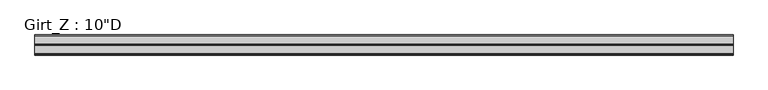
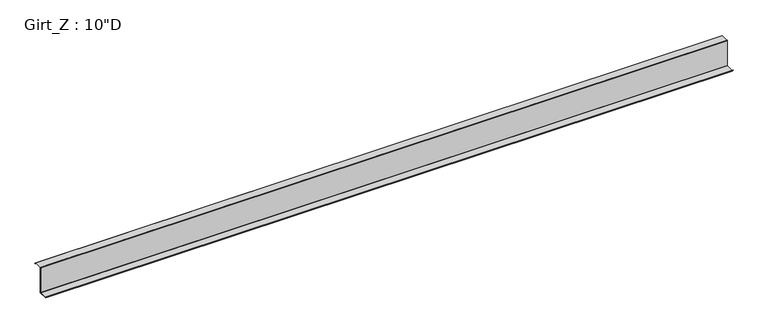
"""IFC4 building model written with IfcOpenShell, lengths in millimetres: beam geometry."""

import ifcopenshell
import ifcopenshell.guid

model = None  # the IFC model being written
_history = None  # IfcOwnerHistory: only IFC2X3 demands one
_inside = {}  # id of a spatial element -> (the spatial element, [elements in it])
_under = {}  # id of a project, library or spatial element -> (it, [spatial elements below it])
_declared = {}  # id of a project -> (the project, [libraries it declares])
_typed = {}  # id of a type object -> (the type object, [elements of that type])
_made_of = {}  # id of a material, layer set ... -> (it, [elements and type objects made of it])


def new_model(schema):
    """Start an empty IFC model of exactly this schema.

    Asked for "IFC4X3", IfcOpenShell would pick the latest addendum, in which some entities
    have other attributes; the version numbers below select the first issue.
    IFC2X3 requires an IfcOwnerHistory on every rooted entity: one is made here for all.
    """
    global model, _history
    if schema == "IFC4X3":
        model = ifcopenshell.file(schema_version=(4, 3, 0, 0))
    else:
        model = ifcopenshell.file(schema=schema)
    _inside.clear()
    _under.clear()
    _declared.clear()
    _typed.clear()
    _made_of.clear()
    _history = None
    if model.schema == "IFC2X3":
        org = make("IfcOrganization", Name="unknown")
        user = make(
            "IfcPersonAndOrganization",
            ThePerson=make("IfcPerson", FamilyName="unknown"),
            TheOrganization=org,
        )
        app = make(
            "IfcApplication",
            ApplicationDeveloper=org,
            Version="unknown",
            ApplicationFullName="unknown",
            ApplicationIdentifier="unknown",
        )
        _history = make(
            "IfcOwnerHistory",
            OwningUser=user,
            OwningApplication=app,
            ChangeAction="ADDED",
            CreationDate=0,
        )
    return model


def make(cls, **values):
    """One entity of the class cls with the attributes given. An attribute that is None is left unset."""
    return model.create_entity(
        cls, **{name: value for name, value in values.items() if value is not None}
    )


def rooted(cls, **values):
    """An entity with a GlobalId (a new one), such as an element, a storey or a relation."""
    return make(cls, GlobalId=ifcopenshell.guid.new(), OwnerHistory=_history, **values)


def si_unit(unit_type, name, prefix=None):
    """IfcSIUnit, for example si_unit("LENGTHUNIT", "METRE", prefix="MILLI")."""
    return make("IfcSIUnit", UnitType=unit_type, Prefix=prefix, Name=name)


def assignment(units):
    """IfcUnitAssignment: the units of a project."""
    return None if units is None else make("IfcUnitAssignment", Units=units)


def point(xyz):
    """IfcCartesianPoint."""
    return None if xyz is None else make("IfcCartesianPoint", Coordinates=xyz)


def direction(xyz):
    """IfcDirection."""
    return None if xyz is None else make("IfcDirection", DirectionRatios=xyz)


def frame(location, z_axis=None, x_axis=None):
    """IfcAxis2Placement3D, a coordinate frame: its origin and axes. An axis left out is left unset."""
    return make(
        "IfcAxis2Placement3D",
        Location=point(location),
        Axis=direction(z_axis),
        RefDirection=direction(x_axis),
    )


def frame_2d(location, x_axis=None):
    """IfcAxis2Placement2D, a coordinate frame in the plane: its origin and x axis."""
    return make(
        "IfcAxis2Placement2D", Location=point(location), RefDirection=direction(x_axis)
    )


def origin():
    """The frame at (0, 0, 0) with its axes left unset."""
    return frame((0.0, 0.0, 0.0))


def place(relative_to, where):
    """IfcLocalPlacement: puts the frame where relative to a parent placement (None: the world)."""
    return make(
        "IfcLocalPlacement", PlacementRelTo=relative_to, RelativePlacement=where
    )


def context(
    kind, dimensions, precision=None, world=None, true_north=None, identifier=None
):
    """IfcGeometricRepresentationContext, for example the 3D "Model" context."""
    return make(
        "IfcGeometricRepresentationContext",
        ContextIdentifier=identifier,
        ContextType=kind,
        CoordinateSpaceDimension=dimensions,
        Precision=precision,
        WorldCoordinateSystem=world,
        TrueNorth=true_north,
    )


def project(units=None, contexts=None):
    """IfcProject with its units and contexts."""
    return rooted(
        "IfcProject",
        Name="project",
        RepresentationContexts=contexts,
        UnitsInContext=assignment(units),
    )


def spatial(cls, under=None, at=None, **own):
    """A site, building, storey or space (cls), placed at a placement, below another one or the project."""
    s = rooted(cls, ObjectPlacement=at, **own)
    if under is not None:
        _under.setdefault(under.id(), (under, []))[1].append(s)
    return s


def polyline(points):
    """IfcPolyline through the points."""
    return make("IfcPolyline", Points=[point(p) for p in points])


def circle_curve(where, radius):
    """IfcCircle in the frame where."""
    return make("IfcCircle", Position=where, Radius=radius)


def trimmed(basis, trim1, trim2, sense, master):
    """IfcTrimmedCurve: the piece of a basis curve between two trims."""
    return make(
        "IfcTrimmedCurve",
        BasisCurve=basis,
        Trim1=trim1,
        Trim2=trim2,
        SenseAgreement=sense,
        MasterRepresentation=master,
    )


def segment(curve, same_sense, transition):
    """IfcCompositeCurveSegment."""
    return make(
        "IfcCompositeCurveSegment",
        Transition=transition,
        SameSense=same_sense,
        ParentCurve=curve,
    )


def composite_curve(segments, self_intersect=None):
    """IfcCompositeCurve: segments joined end to end."""
    return make("IfcCompositeCurve", Segments=segments, SelfIntersect=self_intersect)


def outline(outer, holes=None, kind="AREA"):
    """IfcArbitraryClosedProfileDef: a profile drawn as a closed curve; with holes, ...WithVoids."""
    if holes is None:
        return make("IfcArbitraryClosedProfileDef", ProfileType=kind, OuterCurve=outer)
    return make(
        "IfcArbitraryProfileDefWithVoids",
        ProfileType=kind,
        OuterCurve=outer,
        InnerCurves=holes,
    )


def extrude(swept, where, along, depth):
    """IfcExtrudedAreaSolid: the profile swept, set in the frame where, extruded along a direction by depth."""
    return make(
        "IfcExtrudedAreaSolid",
        SweptArea=swept,
        Position=where,
        ExtrudedDirection=direction(along),
        Depth=depth,
    )


def shape(context_of_items, identifier, shape_type, items):
    """IfcShapeRepresentation: the items that make up one representation, for example the "Body"."""
    return make(
        "IfcShapeRepresentation",
        ContextOfItems=context_of_items,
        RepresentationIdentifier=identifier,
        RepresentationType=shape_type,
        Items=items,
    )


def source(mapping_origin, context_of_items, identifier, shape_type, items):
    """IfcRepresentationMap: a shape defined once, which mapped items show again and again."""
    return make(
        "IfcRepresentationMap",
        MappingOrigin=mapping_origin,
        MappedRepresentation=shape(context_of_items, identifier, shape_type, items),
    )


def transform(
    local_origin,
    x_axis=None,
    y_axis=None,
    z_axis=None,
    scale=None,
    scale2=None,
    scale3=None,
    uniform=True,
):
    """IfcCartesianTransformationOperator3D, or its non-uniform kind. x_axis, y_axis, z_axis: its Axis1, 2, 3."""
    if uniform:
        return make(
            "IfcCartesianTransformationOperator3D",
            Axis1=direction(x_axis),
            Axis2=direction(y_axis),
            LocalOrigin=point(local_origin),
            Scale=scale,
            Axis3=direction(z_axis),
        )
    return make(
        "IfcCartesianTransformationOperator3DnonUniform",
        Axis1=direction(x_axis),
        Axis2=direction(y_axis),
        LocalOrigin=point(local_origin),
        Scale=scale,
        Axis3=direction(z_axis),
        Scale2=scale2,
        Scale3=scale3,
    )


def mapped(mapping_source, mapping_target):
    """IfcMappedItem: shows the shape of a source again, moved by a transform."""
    return make(
        "IfcMappedItem", MappingSource=mapping_source, MappingTarget=mapping_target
    )


def made_of(thing, what):
    """Note that an element or type object is made of a material, layer set ...; save() writes the relation."""
    if what is not None:
        _made_of.setdefault(what.id(), (what, []))[1].append(thing)
    return thing


def element(
    cls,
    number,
    at=None,
    inside=None,
    cuts=None,
    type_object=None,
    material=None,
    context=None,
    identifier="Body",
    shape_type=None,
    held_by="IfcProductDefinitionShape",
    body=None,
    shapes=None,
    **own,
):
    """One element of the class cls, such as IfcWall. Its Tag is "e" and its number.

    at: its placement. inside: the storey or other place that contains it. cuts: it is an
    opening in that element (IfcRelVoidsElement). A single representation is given by context,
    identifier, shape_type and body (its items); several are given by shapes. held_by: the class
    of the entity that holds the representations. save() writes the other relations.
    """
    e = rooted(cls, Tag="e%d" % number, ObjectPlacement=at, **own)
    if body is not None:
        shapes = [shape(context, identifier, shape_type, body)]
    if shapes is not None:
        e.Representation = make(held_by, Representations=shapes)
    if inside is not None:
        _inside.setdefault(inside.id(), (inside, []))[1].append(e)
    if cuts is not None:
        rooted(
            "IfcRelVoidsElement", RelatingBuildingElement=cuts, RelatedOpeningElement=e
        )
    if type_object is not None:
        _typed.setdefault(type_object.id(), (type_object, []))[1].append(e)
    return made_of(e, material)


def aggregate(whole, parts):
    """IfcRelAggregates: a whole, such as a stair, and the parts it consists of."""
    return rooted("IfcRelAggregates", RelatingObject=whole, RelatedObjects=parts)


def save(model, path):
    """Write the relations noted so far, then the file.

    IfcRelAggregates (storeys below a building ...), IfcRelContainedInSpatialStructure (elements
    in a storey), IfcRelDefinesByType, IfcRelAssociatesMaterial and IfcRelDeclares: one each for
    every whole, place, type object, material and project.
    """
    for whole, parts in _under.values():
        aggregate(whole, parts)
    for where, things in _inside.values():
        rooted(
            "IfcRelContainedInSpatialStructure",
            RelatedElements=things,
            RelatingStructure=where,
        )
    for kind, things in _typed.values():
        rooted("IfcRelDefinesByType", RelatedObjects=things, RelatingType=kind)
    for what, things in _made_of.values():
        rooted("IfcRelAssociatesMaterial", RelatedObjects=things, RelatingMaterial=what)
    for by, libraries in _declared.values():
        rooted("IfcRelDeclares", RelatingContext=by, RelatedDefinitions=libraries)
    model.write(path)


def beam_44ace1b0(model_context):
    return source(origin(), model_context, "Body", "SweptSolid", [
        extrude(outline(composite_curve([segment(polyline([(77.9859375, 127.0), (90.2310415, 112.4068534), (88.1028742, 110.621109), (76.6904765, 124.221875), (3.3005807, 124.221875)]), True, "CONTINUOUS"), segment(trimmed(circle_curve(frame_2d((3.3741066, 122.2381931)), 1.9850441), [point((3.3005807, 124.221875))], [point((1.3890625, 122.2381931))], True, "CARTESIAN"), True, "CONTINUOUS"), segment(polyline([(1.3890625, 122.2381931), (1.3890625, -127.0), (-84.3359375, -127.0), (-96.5810415, -112.4068534), (-94.4528742, -110.621109), (-83.0404765, -124.221875), (-3.2694106, -124.221875)]), True, "CONTINUOUS"), segment(trimmed(circle_curve(frame_2d((-3.3748024, -122.2389339)), 1.9857399), [point((-3.2694106, -124.221875))], [point((-1.3890625, -122.2389339))], True, "CARTESIAN"), True, "CONTINUOUS"), segment(polyline([(-1.3890625, -122.2389339), (-1.3890625, 122.2375)]), True, "CONTINUOUS"), segment(trimmed(circle_curve(frame_2d((3.3734375, 122.2375)), 4.7625), [point((-1.3890625, 122.2375))], [point((3.3734375, 127.0))], False, "CARTESIAN"), True, "CONTINUOUS"), segment(polyline([(3.3734375, 127.0), (77.9859375, 127.0)]), True, "CONTINUOUS")], self_intersect=False)), frame((-3314.7, 0.0, 0.0), z_axis=(1.0, 0.0, 0.0), x_axis=(0.0, 1.0, 0.0)), (0.0, 0.0, 1.0), 6470.65),
    ])


if __name__ == "__main__":
    model = new_model("IFC4")
    model_context = context("Model", 3, world=origin())
    ifc_project = project(units=[si_unit("LENGTHUNIT", "METRE", prefix="MILLI")], contexts=[model_context])
    site = spatial("IfcSite", under=ifc_project)
    building = spatial("IfcBuilding", under=site)
    placement = place(None, origin())
    beam_shape = beam_44ace1b0(model_context)
    element("IfcBeam", 1, ObjectType="Girt_Z : 10\"D", at=placement, inside=building, context=model_context, shape_type="MappedRepresentation", body=[
        mapped(beam_shape, transform((0.0, 0.0, 0.0), x_axis=(1.0, 0.0, 0.0), y_axis=(0.0, 1.0, 0.0), z_axis=(0.0, 0.0, 1.0))),
    ])
    save(model, "model.ifc")

# Revit data of these elements
# Type "Girt_Z : 10\"D"
#   half leg = 0' - 1 11/16"
#   Web_Thickness = 0' - 0 7/64"
#   Length [instance default] = 10' - 0"
#   Leg_2 = 0' - 3 3/8"
#   Leg_1 = 0' - 3 1/8"
#   Height = 0' - 10"
#   Structural Material [instance default] = none
# Element 1 (IfcBeam, "Girt_Z : 10\"D")
#   Structural Material = STRUCTURAL STEEL - SEE STRUCT. DWGS
#   Materials on its faces: "STRUCTURAL STEEL - SEE STRUCT. DWGS"
# Materials
#   "STRUCTURAL STEEL - SEE STRUCT. DWGS": class "Metal", colour RGB 137 146 153, transparency 0, Description = "Steel, mill finish", Cost = 0
